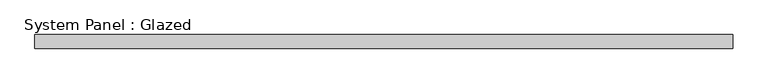
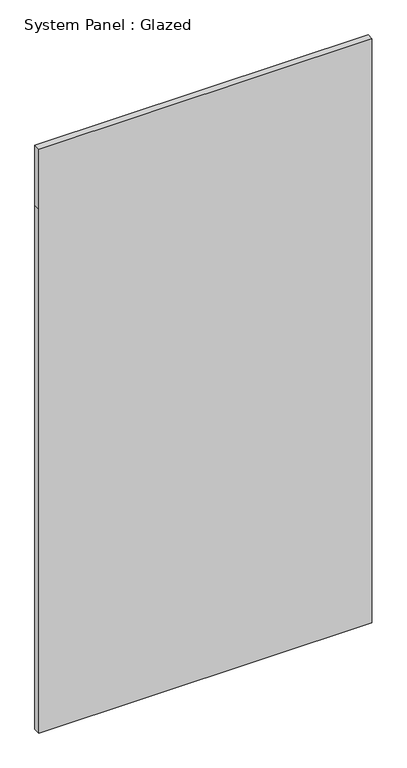
"""IFC4 building model written with IfcOpenShell, lengths in millimetres: plate geometry, System Panel : Glazed."""

from ifc_helpers import new_model, si_unit, frame, origin, place, context, project, spatial, polyline, outline, extrude, source, transform, mapped, element, save


def system_panel_glazed_6ed60089(model_context):
    return source(origin(), model_context, "Body", "SweptSolid", [
        extrude(outline(polyline([(0.0, -632.2785714), (0.0, 632.2785714), (2101.85, 632.2785714), (2343.15, 632.2785714), (2343.15, -632.2785714), (2101.85, -632.2785714), (0.0, -632.2785714)])), frame((0.0, 19.05, 0.0), z_axis=(0.0, 1.0, 0.0), x_axis=(0.0, 0.0, 1.0)), (0.0, 0.0, 1.0), 25.4),
    ])


if __name__ == "__main__":
    model = new_model("IFC4")
    model_context = context("Model", 3, world=origin())
    ifc_project = project(units=[si_unit("LENGTHUNIT", "METRE", prefix="MILLI")], contexts=[model_context])
    site = spatial("IfcSite", under=ifc_project)
    building = spatial("IfcBuilding", under=site)
    placement = place(None, origin())
    system_panel_glazed_shape = system_panel_glazed_6ed60089(model_context)
    element("IfcPlate", 1, ObjectType="System Panel : Glazed", at=placement, inside=building, context=model_context, shape_type="MappedRepresentation", body=[
        mapped(system_panel_glazed_shape, transform((0.0, 0.0, 0.0), x_axis=(1.0, 0.0, 0.0), y_axis=(0.0, 1.0, 0.0), z_axis=(0.0, 0.0, 1.0))),
    ])
    save(model, "model.ifc")

# Revit data of these elements
# Element 1 (IfcPlate, "System Panel : Glazed")
#   Materials on its faces: "Glass"
# Materials
#   "Glass": class "Glass", colour RGB 0 128 192, transparency 0.75
